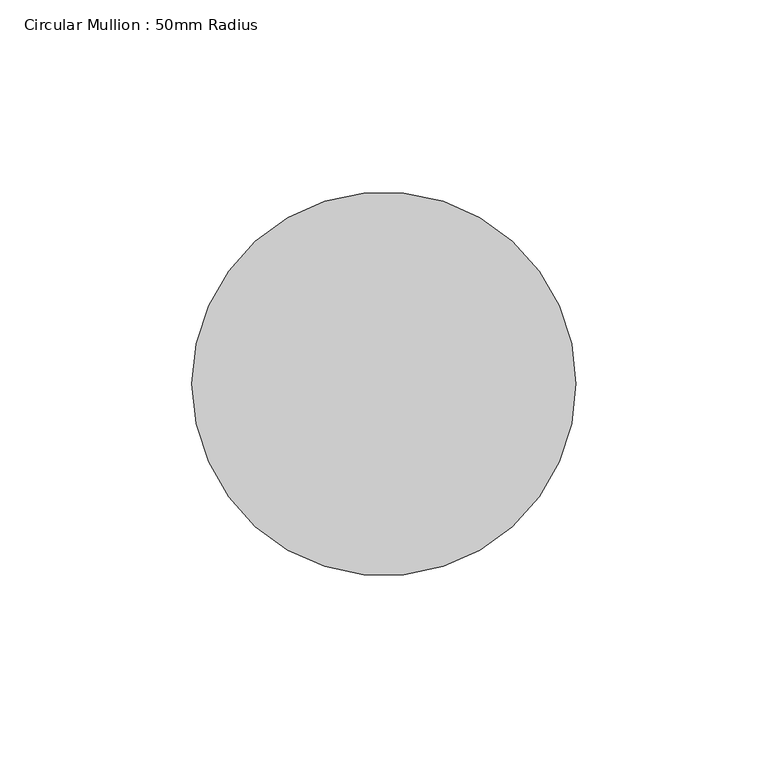
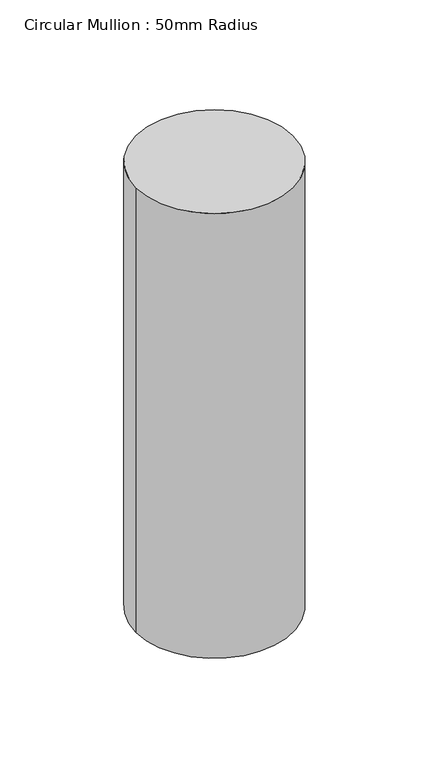
"""IFC4 building model written with IfcOpenShell, lengths in millimetres: member geometry, Circular Mullion : 50mm Radius."""

import ifcopenshell
import ifcopenshell.guid

model = None  # the IFC model being written
_history = None  # IfcOwnerHistory: only IFC2X3 demands one
_inside = {}  # id of a spatial element -> (the spatial element, [elements in it])
_under = {}  # id of a project, library or spatial element -> (it, [spatial elements below it])
_declared = {}  # id of a project -> (the project, [libraries it declares])
_typed = {}  # id of a type object -> (the type object, [elements of that type])
_made_of = {}  # id of a material, layer set ... -> (it, [elements and type objects made of it])


def new_model(schema):
    """Start an empty IFC model of exactly this schema.

    Asked for "IFC4X3", IfcOpenShell would pick the latest addendum, in which some entities
    have other attributes; the version numbers below select the first issue.
    IFC2X3 requires an IfcOwnerHistory on every rooted entity: one is made here for all.
    """
    global model, _history
    if schema == "IFC4X3":
        model = ifcopenshell.file(schema_version=(4, 3, 0, 0))
    else:
        model = ifcopenshell.file(schema=schema)
    _inside.clear()
    _under.clear()
    _declared.clear()
    _typed.clear()
    _made_of.clear()
    _history = None
    if model.schema == "IFC2X3":
        org = make("IfcOrganization", Name="unknown")
        user = make(
            "IfcPersonAndOrganization",
            ThePerson=make("IfcPerson", FamilyName="unknown"),
            TheOrganization=org,
        )
        app = make(
            "IfcApplication",
            ApplicationDeveloper=org,
            Version="unknown",
            ApplicationFullName="unknown",
            ApplicationIdentifier="unknown",
        )
        _history = make(
            "IfcOwnerHistory",
            OwningUser=user,
            OwningApplication=app,
            ChangeAction="ADDED",
            CreationDate=0,
        )
    return model


def make(cls, **values):
    """One entity of the class cls with the attributes given. An attribute that is None is left unset."""
    return model.create_entity(
        cls, **{name: value for name, value in values.items() if value is not None}
    )


def rooted(cls, **values):
    """An entity with a GlobalId (a new one), such as an element, a storey or a relation."""
    return make(cls, GlobalId=ifcopenshell.guid.new(), OwnerHistory=_history, **values)


def si_unit(unit_type, name, prefix=None):
    """IfcSIUnit, for example si_unit("LENGTHUNIT", "METRE", prefix="MILLI")."""
    return make("IfcSIUnit", UnitType=unit_type, Prefix=prefix, Name=name)


def assignment(units):
    """IfcUnitAssignment: the units of a project."""
    return None if units is None else make("IfcUnitAssignment", Units=units)


def point(xyz):
    """IfcCartesianPoint."""
    return None if xyz is None else make("IfcCartesianPoint", Coordinates=xyz)


def direction(xyz):
    """IfcDirection."""
    return None if xyz is None else make("IfcDirection", DirectionRatios=xyz)


def frame(location, z_axis=None, x_axis=None):
    """IfcAxis2Placement3D, a coordinate frame: its origin and axes. An axis left out is left unset."""
    return make(
        "IfcAxis2Placement3D",
        Location=point(location),
        Axis=direction(z_axis),
        RefDirection=direction(x_axis),
    )


def frame_2d(location, x_axis=None):
    """IfcAxis2Placement2D, a coordinate frame in the plane: its origin and x axis."""
    return make(
        "IfcAxis2Placement2D", Location=point(location), RefDirection=direction(x_axis)
    )


def origin():
    """The frame at (0, 0, 0) with its axes left unset."""
    return frame((0.0, 0.0, 0.0))


def origin_2d():
    """The frame at (0, 0) in the plane with its x axis left unset."""
    return frame_2d((0.0, 0.0))


def place(relative_to, where):
    """IfcLocalPlacement: puts the frame where relative to a parent placement (None: the world)."""
    return make(
        "IfcLocalPlacement", PlacementRelTo=relative_to, RelativePlacement=where
    )


def context(
    kind, dimensions, precision=None, world=None, true_north=None, identifier=None
):
    """IfcGeometricRepresentationContext, for example the 3D "Model" context."""
    return make(
        "IfcGeometricRepresentationContext",
        ContextIdentifier=identifier,
        ContextType=kind,
        CoordinateSpaceDimension=dimensions,
        Precision=precision,
        WorldCoordinateSystem=world,
        TrueNorth=true_north,
    )


def project(units=None, contexts=None):
    """IfcProject with its units and contexts."""
    return rooted(
        "IfcProject",
        Name="project",
        RepresentationContexts=contexts,
        UnitsInContext=assignment(units),
    )


def spatial(cls, under=None, at=None, **own):
    """A site, building, storey or space (cls), placed at a placement, below another one or the project."""
    s = rooted(cls, ObjectPlacement=at, **own)
    if under is not None:
        _under.setdefault(under.id(), (under, []))[1].append(s)
    return s


def circle_curve(where, radius):
    """IfcCircle in the frame where."""
    return make("IfcCircle", Position=where, Radius=radius)


def trimmed(basis, trim1, trim2, sense, master):
    """IfcTrimmedCurve: the piece of a basis curve between two trims."""
    return make(
        "IfcTrimmedCurve",
        BasisCurve=basis,
        Trim1=trim1,
        Trim2=trim2,
        SenseAgreement=sense,
        MasterRepresentation=master,
    )


def segment(curve, same_sense, transition):
    """IfcCompositeCurveSegment."""
    return make(
        "IfcCompositeCurveSegment",
        Transition=transition,
        SameSense=same_sense,
        ParentCurve=curve,
    )


def composite_curve(segments, self_intersect=None):
    """IfcCompositeCurve: segments joined end to end."""
    return make("IfcCompositeCurve", Segments=segments, SelfIntersect=self_intersect)


def outline(outer, holes=None, kind="AREA"):
    """IfcArbitraryClosedProfileDef: a profile drawn as a closed curve; with holes, ...WithVoids."""
    if holes is None:
        return make("IfcArbitraryClosedProfileDef", ProfileType=kind, OuterCurve=outer)
    return make(
        "IfcArbitraryProfileDefWithVoids",
        ProfileType=kind,
        OuterCurve=outer,
        InnerCurves=holes,
    )


def extrude(swept, where, along, depth):
    """IfcExtrudedAreaSolid: the profile swept, set in the frame where, extruded along a direction by depth."""
    return make(
        "IfcExtrudedAreaSolid",
        SweptArea=swept,
        Position=where,
        ExtrudedDirection=direction(along),
        Depth=depth,
    )


def shape(context_of_items, identifier, shape_type, items):
    """IfcShapeRepresentation: the items that make up one representation, for example the "Body"."""
    return make(
        "IfcShapeRepresentation",
        ContextOfItems=context_of_items,
        RepresentationIdentifier=identifier,
        RepresentationType=shape_type,
        Items=items,
    )


def source(mapping_origin, context_of_items, identifier, shape_type, items):
    """IfcRepresentationMap: a shape defined once, which mapped items show again and again."""
    return make(
        "IfcRepresentationMap",
        MappingOrigin=mapping_origin,
        MappedRepresentation=shape(context_of_items, identifier, shape_type, items),
    )


def transform(
    local_origin,
    x_axis=None,
    y_axis=None,
    z_axis=None,
    scale=None,
    scale2=None,
    scale3=None,
    uniform=True,
):
    """IfcCartesianTransformationOperator3D, or its non-uniform kind. x_axis, y_axis, z_axis: its Axis1, 2, 3."""
    if uniform:
        return make(
            "IfcCartesianTransformationOperator3D",
            Axis1=direction(x_axis),
            Axis2=direction(y_axis),
            LocalOrigin=point(local_origin),
            Scale=scale,
            Axis3=direction(z_axis),
        )
    return make(
        "IfcCartesianTransformationOperator3DnonUniform",
        Axis1=direction(x_axis),
        Axis2=direction(y_axis),
        LocalOrigin=point(local_origin),
        Scale=scale,
        Axis3=direction(z_axis),
        Scale2=scale2,
        Scale3=scale3,
    )


def mapped(mapping_source, mapping_target):
    """IfcMappedItem: shows the shape of a source again, moved by a transform."""
    return make(
        "IfcMappedItem", MappingSource=mapping_source, MappingTarget=mapping_target
    )


def made_of(thing, what):
    """Note that an element or type object is made of a material, layer set ...; save() writes the relation."""
    if what is not None:
        _made_of.setdefault(what.id(), (what, []))[1].append(thing)
    return thing


def element(
    cls,
    number,
    at=None,
    inside=None,
    cuts=None,
    type_object=None,
    material=None,
    context=None,
    identifier="Body",
    shape_type=None,
    held_by="IfcProductDefinitionShape",
    body=None,
    shapes=None,
    **own,
):
    """One element of the class cls, such as IfcWall. Its Tag is "e" and its number.

    at: its placement. inside: the storey or other place that contains it. cuts: it is an
    opening in that element (IfcRelVoidsElement). A single representation is given by context,
    identifier, shape_type and body (its items); several are given by shapes. held_by: the class
    of the entity that holds the representations. save() writes the other relations.
    """
    e = rooted(cls, Tag="e%d" % number, ObjectPlacement=at, **own)
    if body is not None:
        shapes = [shape(context, identifier, shape_type, body)]
    if shapes is not None:
        e.Representation = make(held_by, Representations=shapes)
    if inside is not None:
        _inside.setdefault(inside.id(), (inside, []))[1].append(e)
    if cuts is not None:
        rooted(
            "IfcRelVoidsElement", RelatingBuildingElement=cuts, RelatedOpeningElement=e
        )
    if type_object is not None:
        _typed.setdefault(type_object.id(), (type_object, []))[1].append(e)
    return made_of(e, material)


def aggregate(whole, parts):
    """IfcRelAggregates: a whole, such as a stair, and the parts it consists of."""
    return rooted("IfcRelAggregates", RelatingObject=whole, RelatedObjects=parts)


def save(model, path):
    """Write the relations noted so far, then the file.

    IfcRelAggregates (storeys below a building ...), IfcRelContainedInSpatialStructure (elements
    in a storey), IfcRelDefinesByType, IfcRelAssociatesMaterial and IfcRelDeclares: one each for
    every whole, place, type object, material and project.
    """
    for whole, parts in _under.values():
        aggregate(whole, parts)
    for where, things in _inside.values():
        rooted(
            "IfcRelContainedInSpatialStructure",
            RelatedElements=things,
            RelatingStructure=where,
        )
    for kind, things in _typed.values():
        rooted("IfcRelDefinesByType", RelatedObjects=things, RelatingType=kind)
    for what, things in _made_of.values():
        rooted("IfcRelAssociatesMaterial", RelatedObjects=things, RelatingMaterial=what)
    for by, libraries in _declared.values():
        rooted("IfcRelDeclares", RelatingContext=by, RelatedDefinitions=libraries)
    model.write(path)


def circular_mullion_50mm_radius_ecc39a4c(model_context):
    return source(origin(), model_context, "Body", "SweptSolid", [
        extrude(outline(composite_curve([segment(trimmed(circle_curve(origin_2d(), 50.0), [point((50.0, 0.0))], [point((-50.0, 0.0))], False, "CARTESIAN"), True, "CONTINUOUS"), segment(trimmed(circle_curve(origin_2d(), 50.0), [point((-50.0, 0.0))], [point((50.0, 0.0))], False, "CARTESIAN"), True, "CONTINUOUS")], self_intersect=False)), frame((0.0, 0.0, -299.5043756), z_axis=(0.0, 0.0, 1.0), x_axis=(1.0, 0.0, 0.0)), (0.0, 0.0, 1.0), 299.5043756),
    ])


if __name__ == "__main__":
    model = new_model("IFC4")
    model_context = context("Model", 3, world=origin())
    ifc_project = project(units=[si_unit("LENGTHUNIT", "METRE", prefix="MILLI")], contexts=[model_context])
    site = spatial("IfcSite", under=ifc_project)
    building = spatial("IfcBuilding", under=site)
    placement = place(None, origin())
    circular_mullion_50mm_radius_shape = circular_mullion_50mm_radius_ecc39a4c(model_context)
    element("IfcMember", 1, ObjectType="Circular Mullion : 50mm Radius", at=placement, inside=building, context=model_context, shape_type="MappedRepresentation", body=[
        mapped(circular_mullion_50mm_radius_shape, transform((0.0, 0.0, 0.0), x_axis=(1.0, 0.0, 0.0), y_axis=(0.0, 1.0, 0.0), z_axis=(0.0, 0.0, 1.0))),
    ])
    save(model, "model.ifc")

# Revit data of these elements
# Type "Circular Mullion : 50mm Radius"
#   built-in parameter 1007350 = 0.164042 (stored number, unit not read)
# Element 1 (IfcMember, "Circular Mullion : 50mm Radius")
#   Materials on its faces: "Aluminium"
# Materials
#   "Aluminium": class "Metal", colour RGB 247 247 247, transparency 0, Description = "Aluminium 6061", Cost = 0
